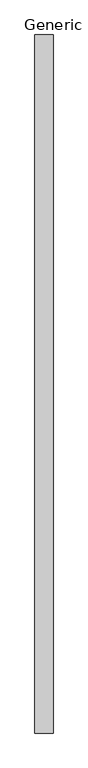
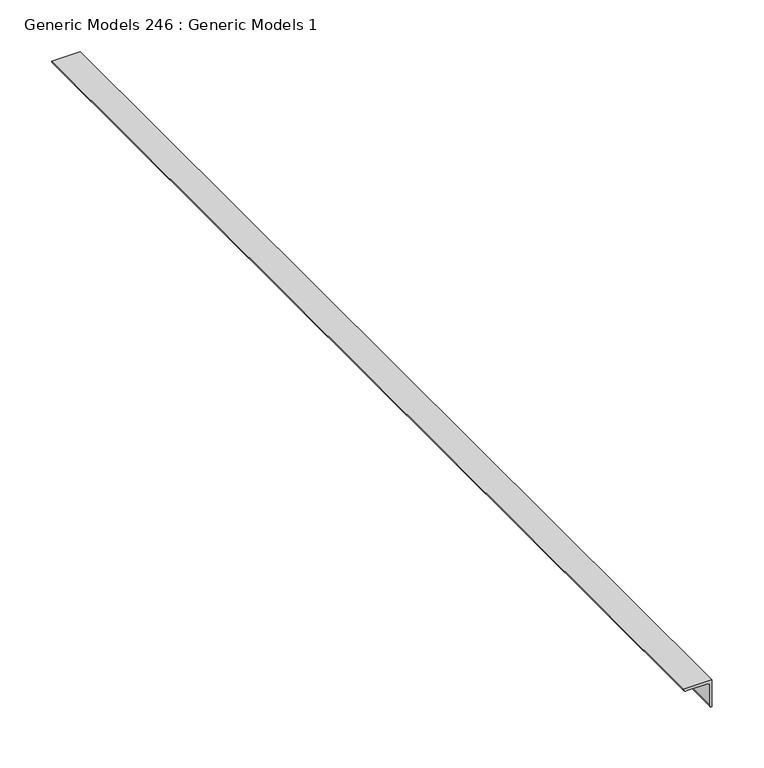
"""IFC4 building model written with IfcOpenShell, lengths in millimetres: proxy geometry, Generic Models 246 : Generic Models 1."""

import ifcopenshell
import ifcopenshell.guid

model = None  # the IFC model being written
_history = None  # IfcOwnerHistory: only IFC2X3 demands one
_inside = {}  # id of a spatial element -> (the spatial element, [elements in it])
_under = {}  # id of a project, library or spatial element -> (it, [spatial elements below it])
_declared = {}  # id of a project -> (the project, [libraries it declares])
_typed = {}  # id of a type object -> (the type object, [elements of that type])
_made_of = {}  # id of a material, layer set ... -> (it, [elements and type objects made of it])


def new_model(schema):
    """Start an empty IFC model of exactly this schema.

    Asked for "IFC4X3", IfcOpenShell would pick the latest addendum, in which some entities
    have other attributes; the version numbers below select the first issue.
    IFC2X3 requires an IfcOwnerHistory on every rooted entity: one is made here for all.
    """
    global model, _history
    if schema == "IFC4X3":
        model = ifcopenshell.file(schema_version=(4, 3, 0, 0))
    else:
        model = ifcopenshell.file(schema=schema)
    _inside.clear()
    _under.clear()
    _declared.clear()
    _typed.clear()
    _made_of.clear()
    _history = None
    if model.schema == "IFC2X3":
        org = make("IfcOrganization", Name="unknown")
        user = make(
            "IfcPersonAndOrganization",
            ThePerson=make("IfcPerson", FamilyName="unknown"),
            TheOrganization=org,
        )
        app = make(
            "IfcApplication",
            ApplicationDeveloper=org,
            Version="unknown",
            ApplicationFullName="unknown",
            ApplicationIdentifier="unknown",
        )
        _history = make(
            "IfcOwnerHistory",
            OwningUser=user,
            OwningApplication=app,
            ChangeAction="ADDED",
            CreationDate=0,
        )
    return model


def make(cls, **values):
    """One entity of the class cls with the attributes given. An attribute that is None is left unset."""
    return model.create_entity(
        cls, **{name: value for name, value in values.items() if value is not None}
    )


def rooted(cls, **values):
    """An entity with a GlobalId (a new one), such as an element, a storey or a relation."""
    return make(cls, GlobalId=ifcopenshell.guid.new(), OwnerHistory=_history, **values)


def si_unit(unit_type, name, prefix=None):
    """IfcSIUnit, for example si_unit("LENGTHUNIT", "METRE", prefix="MILLI")."""
    return make("IfcSIUnit", UnitType=unit_type, Prefix=prefix, Name=name)


def assignment(units):
    """IfcUnitAssignment: the units of a project."""
    return None if units is None else make("IfcUnitAssignment", Units=units)


def point(xyz):
    """IfcCartesianPoint."""
    return None if xyz is None else make("IfcCartesianPoint", Coordinates=xyz)


def direction(xyz):
    """IfcDirection."""
    return None if xyz is None else make("IfcDirection", DirectionRatios=xyz)


def frame(location, z_axis=None, x_axis=None):
    """IfcAxis2Placement3D, a coordinate frame: its origin and axes. An axis left out is left unset."""
    return make(
        "IfcAxis2Placement3D",
        Location=point(location),
        Axis=direction(z_axis),
        RefDirection=direction(x_axis),
    )


def frame_2d(location, x_axis=None):
    """IfcAxis2Placement2D, a coordinate frame in the plane: its origin and x axis."""
    return make(
        "IfcAxis2Placement2D", Location=point(location), RefDirection=direction(x_axis)
    )


def origin():
    """The frame at (0, 0, 0) with its axes left unset."""
    return frame((0.0, 0.0, 0.0))


def place(relative_to, where):
    """IfcLocalPlacement: puts the frame where relative to a parent placement (None: the world)."""
    return make(
        "IfcLocalPlacement", PlacementRelTo=relative_to, RelativePlacement=where
    )


def context(
    kind, dimensions, precision=None, world=None, true_north=None, identifier=None
):
    """IfcGeometricRepresentationContext, for example the 3D "Model" context."""
    return make(
        "IfcGeometricRepresentationContext",
        ContextIdentifier=identifier,
        ContextType=kind,
        CoordinateSpaceDimension=dimensions,
        Precision=precision,
        WorldCoordinateSystem=world,
        TrueNorth=true_north,
    )


def project(units=None, contexts=None):
    """IfcProject with its units and contexts."""
    return rooted(
        "IfcProject",
        Name="project",
        RepresentationContexts=contexts,
        UnitsInContext=assignment(units),
    )


def spatial(cls, under=None, at=None, **own):
    """A site, building, storey or space (cls), placed at a placement, below another one or the project."""
    s = rooted(cls, ObjectPlacement=at, **own)
    if under is not None:
        _under.setdefault(under.id(), (under, []))[1].append(s)
    return s


def polyline(points):
    """IfcPolyline through the points."""
    return make("IfcPolyline", Points=[point(p) for p in points])


def circle_curve(where, radius):
    """IfcCircle in the frame where."""
    return make("IfcCircle", Position=where, Radius=radius)


def trimmed(basis, trim1, trim2, sense, master):
    """IfcTrimmedCurve: the piece of a basis curve between two trims."""
    return make(
        "IfcTrimmedCurve",
        BasisCurve=basis,
        Trim1=trim1,
        Trim2=trim2,
        SenseAgreement=sense,
        MasterRepresentation=master,
    )


def segment(curve, same_sense, transition):
    """IfcCompositeCurveSegment."""
    return make(
        "IfcCompositeCurveSegment",
        Transition=transition,
        SameSense=same_sense,
        ParentCurve=curve,
    )


def composite_curve(segments, self_intersect=None):
    """IfcCompositeCurve: segments joined end to end."""
    return make("IfcCompositeCurve", Segments=segments, SelfIntersect=self_intersect)


def outline(outer, holes=None, kind="AREA"):
    """IfcArbitraryClosedProfileDef: a profile drawn as a closed curve; with holes, ...WithVoids."""
    if holes is None:
        return make("IfcArbitraryClosedProfileDef", ProfileType=kind, OuterCurve=outer)
    return make(
        "IfcArbitraryProfileDefWithVoids",
        ProfileType=kind,
        OuterCurve=outer,
        InnerCurves=holes,
    )


def extrude(swept, where, along, depth):
    """IfcExtrudedAreaSolid: the profile swept, set in the frame where, extruded along a direction by depth."""
    return make(
        "IfcExtrudedAreaSolid",
        SweptArea=swept,
        Position=where,
        ExtrudedDirection=direction(along),
        Depth=depth,
    )


def shape(context_of_items, identifier, shape_type, items):
    """IfcShapeRepresentation: the items that make up one representation, for example the "Body"."""
    return make(
        "IfcShapeRepresentation",
        ContextOfItems=context_of_items,
        RepresentationIdentifier=identifier,
        RepresentationType=shape_type,
        Items=items,
    )


def source(mapping_origin, context_of_items, identifier, shape_type, items):
    """IfcRepresentationMap: a shape defined once, which mapped items show again and again."""
    return make(
        "IfcRepresentationMap",
        MappingOrigin=mapping_origin,
        MappedRepresentation=shape(context_of_items, identifier, shape_type, items),
    )


def transform(
    local_origin,
    x_axis=None,
    y_axis=None,
    z_axis=None,
    scale=None,
    scale2=None,
    scale3=None,
    uniform=True,
):
    """IfcCartesianTransformationOperator3D, or its non-uniform kind. x_axis, y_axis, z_axis: its Axis1, 2, 3."""
    if uniform:
        return make(
            "IfcCartesianTransformationOperator3D",
            Axis1=direction(x_axis),
            Axis2=direction(y_axis),
            LocalOrigin=point(local_origin),
            Scale=scale,
            Axis3=direction(z_axis),
        )
    return make(
        "IfcCartesianTransformationOperator3DnonUniform",
        Axis1=direction(x_axis),
        Axis2=direction(y_axis),
        LocalOrigin=point(local_origin),
        Scale=scale,
        Axis3=direction(z_axis),
        Scale2=scale2,
        Scale3=scale3,
    )


def mapped(mapping_source, mapping_target):
    """IfcMappedItem: shows the shape of a source again, moved by a transform."""
    return make(
        "IfcMappedItem", MappingSource=mapping_source, MappingTarget=mapping_target
    )


def made_of(thing, what):
    """Note that an element or type object is made of a material, layer set ...; save() writes the relation."""
    if what is not None:
        _made_of.setdefault(what.id(), (what, []))[1].append(thing)
    return thing


def element(
    cls,
    number,
    at=None,
    inside=None,
    cuts=None,
    type_object=None,
    material=None,
    context=None,
    identifier="Body",
    shape_type=None,
    held_by="IfcProductDefinitionShape",
    body=None,
    shapes=None,
    **own,
):
    """One element of the class cls, such as IfcWall. Its Tag is "e" and its number.

    at: its placement. inside: the storey or other place that contains it. cuts: it is an
    opening in that element (IfcRelVoidsElement). A single representation is given by context,
    identifier, shape_type and body (its items); several are given by shapes. held_by: the class
    of the entity that holds the representations. save() writes the other relations.
    """
    e = rooted(cls, Tag="e%d" % number, ObjectPlacement=at, **own)
    if body is not None:
        shapes = [shape(context, identifier, shape_type, body)]
    if shapes is not None:
        e.Representation = make(held_by, Representations=shapes)
    if inside is not None:
        _inside.setdefault(inside.id(), (inside, []))[1].append(e)
    if cuts is not None:
        rooted(
            "IfcRelVoidsElement", RelatingBuildingElement=cuts, RelatedOpeningElement=e
        )
    if type_object is not None:
        _typed.setdefault(type_object.id(), (type_object, []))[1].append(e)
    return made_of(e, material)


def aggregate(whole, parts):
    """IfcRelAggregates: a whole, such as a stair, and the parts it consists of."""
    return rooted("IfcRelAggregates", RelatingObject=whole, RelatedObjects=parts)


def save(model, path):
    """Write the relations noted so far, then the file.

    IfcRelAggregates (storeys below a building ...), IfcRelContainedInSpatialStructure (elements
    in a storey), IfcRelDefinesByType, IfcRelAssociatesMaterial and IfcRelDeclares: one each for
    every whole, place, type object, material and project.
    """
    for whole, parts in _under.values():
        aggregate(whole, parts)
    for where, things in _inside.values():
        rooted(
            "IfcRelContainedInSpatialStructure",
            RelatedElements=things,
            RelatingStructure=where,
        )
    for kind, things in _typed.values():
        rooted("IfcRelDefinesByType", RelatedObjects=things, RelatingType=kind)
    for what, things in _made_of.values():
        rooted("IfcRelAssociatesMaterial", RelatedObjects=things, RelatingMaterial=what)
    for by, libraries in _declared.values():
        rooted("IfcRelDeclares", RelatingContext=by, RelatedDefinitions=libraries)
    model.write(path)


def generic_models_246_generic_models_1_33f707d8(model_context):
    return source(origin(), model_context, "Body", "SweptSolid", [
        extrude(outline(composite_curve([segment(polyline([(4267.2, 47363.0625), (4267.2, 47331.3125)]), True, "CONTINUOUS"), segment(trimmed(circle_curve(frame_2d((4267.2, 47334.4875)), 3.175), [point((4267.2, 47331.3125))], [point((4264.025, 47334.4875))], False, "CARTESIAN"), True, "CONTINUOUS"), segment(polyline([(4264.025, 47334.4875), (4264.025, 47358.3)]), True, "CONTINUOUS"), segment(trimmed(circle_curve(frame_2d((4262.4375, 47358.3)), 1.5875), [point((4264.025, 47358.3))], [point((4262.4375, 47359.8875))], True, "CARTESIAN"), True, "CONTINUOUS"), segment(polyline([(4262.4375, 47359.8875), (4238.625, 47359.8875)]), True, "CONTINUOUS"), segment(trimmed(circle_curve(frame_2d((4238.625, 47363.0625)), 3.175), [point((4238.625, 47359.8875))], [point((4235.45, 47363.0625))], False, "CARTESIAN"), True, "CONTINUOUS"), segment(polyline([(4235.45, 47363.0625), (4267.2, 47363.0625)]), True, "CONTINUOUS")], self_intersect=False)), frame((0.0, 0.0, 0.0), z_axis=(0.0, 1.0, 0.0), x_axis=(0.0, 0.0, 1.0)), (0.0, 0.0, 1.0), 1219.2),
    ])


if __name__ == "__main__":
    model = new_model("IFC4")
    model_context = context("Model", 3, world=origin())
    ifc_project = project(units=[si_unit("LENGTHUNIT", "METRE", prefix="MILLI")], contexts=[model_context])
    site = spatial("IfcSite", under=ifc_project)
    building = spatial("IfcBuilding", under=site)
    placement = place(None, origin())
    generic_models_246_generic_models_1_shape = generic_models_246_generic_models_1_33f707d8(model_context)
    element("IfcBuildingElementProxy", 1, Name="Generic Models 246 : Generic Models 1", ObjectType="Generic Models 246 : Generic Models 1", at=placement, inside=building, context=model_context, shape_type="MappedRepresentation", body=[
        mapped(generic_models_246_generic_models_1_shape, transform((0.0, 0.0, 0.0), x_axis=(1.0, 0.0, 0.0), y_axis=(0.0, 1.0, 0.0), z_axis=(0.0, 0.0, 1.0))),
    ])
    save(model, "model.ifc")

# Revit data of these elements
# Element 1 (IfcBuildingElementProxy, "Generic Models 246 : Generic Models 1")
#   Materials on its faces: "BULKHEAD FRAME WORK"
# Materials
#   "BULKHEAD FRAME WORK": class "Metal", colour RGB 189 187 185, transparency 0, Description = "Structural steel 50ksi", Cost = 0
